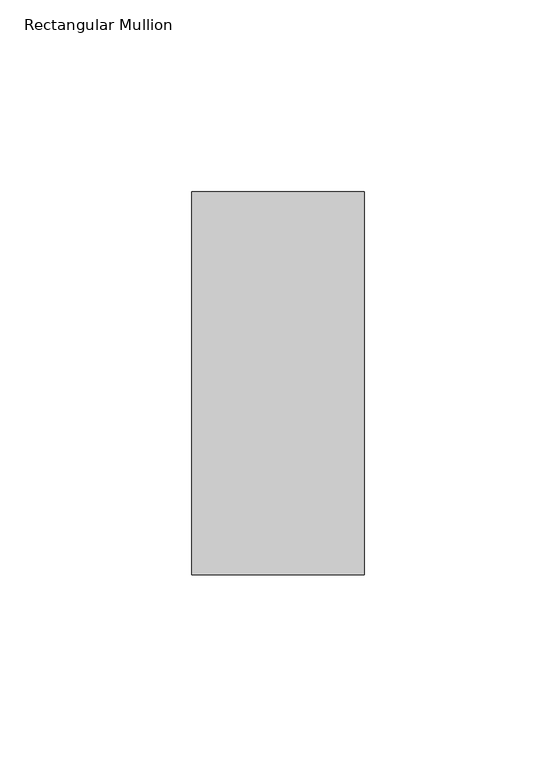
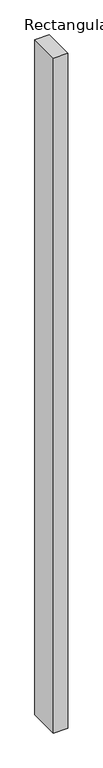
"""IFC4 building model written with IfcOpenShell, lengths in millimetres: member geometry, Rectangular Mullion : 알루미늄_Rectangular Cap_100 x 45."""

from ifc_helpers import new_model, si_unit, frame, origin, place, context, project, spatial, polyline, outline, extrude, source, transform, mapped, element, save


def rectangular_mullion_3ef7a803(model_context):
    return source(origin(), model_context, "Body", "SweptSolid", [
        extrude(outline(polyline([(22.5, 50.0), (22.5, -50.0), (-22.5, -50.0), (-22.5, 50.0), (22.5, 50.0)])), frame((0.0, 0.0, -2222.5), z_axis=(0.0, 0.0, 1.0), x_axis=(1.0, 0.0, 0.0)), (0.0, 0.0, 1.0), 2222.5),
    ])


if __name__ == "__main__":
    model = new_model("IFC4")
    model_context = context("Model", 3, world=origin())
    ifc_project = project(units=[si_unit("LENGTHUNIT", "METRE", prefix="MILLI")], contexts=[model_context])
    site = spatial("IfcSite", under=ifc_project)
    building = spatial("IfcBuilding", under=site)
    placement = place(None, origin())
    rectangular_mullion_shape = rectangular_mullion_3ef7a803(model_context)
    element("IfcMember", 1, ObjectType="Rectangular Mullion : 알루미늄_Rectangular Cap_100 x 45", at=placement, inside=building, context=model_context, shape_type="MappedRepresentation", body=[
        mapped(rectangular_mullion_shape, transform((0.0, 0.0, 0.0), x_axis=(1.0, 0.0, 0.0), y_axis=(0.0, 1.0, 0.0), z_axis=(0.0, 0.0, 1.0))),
    ])
    save(model, "model.ifc")

# Revit data of these elements
# Type "Rectangular Mullion : 알루미늄_Rectangular Cap_100 x 45"
#   built-in parameter 1007304 = 0.328084 (stored number, unit not read)
#   built-in parameter 1007301 = 0.0738189 (stored number, unit not read)
#   built-in parameter 1007300 = 0.0738189 (stored number, unit not read)
# Element 1 (IfcMember, "Rectangular Mullion : 알루미늄_Rectangular Cap_100 x 45")
#   Materials on its faces: "00_Metal_Stainless Steel"
# Materials
#   "00_Metal_Stainless Steel": class "Metal", colour RGB 148 148 148, transparency 0, Description = "Steel", Cost = 0
